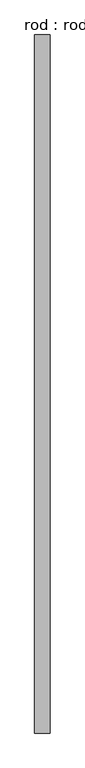
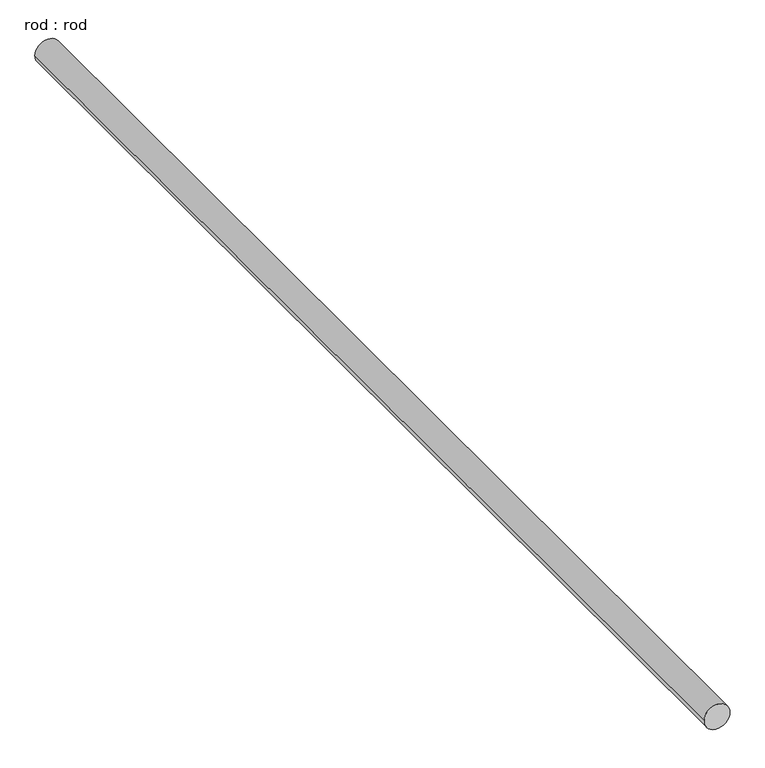
"""IFC4 building model written with IfcOpenShell, lengths in millimetres: proxy geometry, rod : rod."""

from ifc_helpers import new_model, si_unit, point, frame, frame_2d, origin, place, context, project, spatial, circle_curve, trimmed, segment, composite_curve, outline, extrude, source, transform, mapped, element, save


def rod_rod_cc697f86(model_context):
    return source(origin(), model_context, "Body", "SweptSolid", [
        extrude(outline(composite_curve([segment(trimmed(circle_curve(frame_2d((0.0108462, 0.0)), 200.0), [point((0.0108462, 200.0))], [point((0.0108462, -200.0))], False, "CARTESIAN"), True, "CONTINUOUS"), segment(trimmed(circle_curve(frame_2d((0.0108462, 0.0)), 200.0), [point((0.0108462, -200.0))], [point((0.0108462, 200.0))], False, "CARTESIAN"), True, "CONTINUOUS")], self_intersect=False)), frame((0.0, -4892.5124081, 0.0), z_axis=(0.0, 1.0, 0.0), x_axis=(0.0, 0.0, 1.0)), (0.0, 0.0, 1.0), 17970.482047),
    ])


if __name__ == "__main__":
    model = new_model("IFC4")
    model_context = context("Model", 3, world=origin())
    ifc_project = project(units=[si_unit("LENGTHUNIT", "METRE", prefix="MILLI")], contexts=[model_context])
    site = spatial("IfcSite", under=ifc_project)
    building = spatial("IfcBuilding", under=site)
    placement = place(None, origin())
    rod_rod_shape = rod_rod_cc697f86(model_context)
    element("IfcBuildingElementProxy", 1, Name="rod : rod", ObjectType="rod : rod", at=placement, inside=building, context=model_context, shape_type="MappedRepresentation", body=[
        mapped(rod_rod_shape, transform((0.0, 0.0, 0.0), x_axis=(1.0, 0.0, 0.0), y_axis=(0.0, 1.0, 0.0), z_axis=(0.0, 0.0, 1.0))),
    ])
    save(model, "model.ifc")

# Revit data of these elements
# Type "rod : rod"
#   Default Elevation = 0
